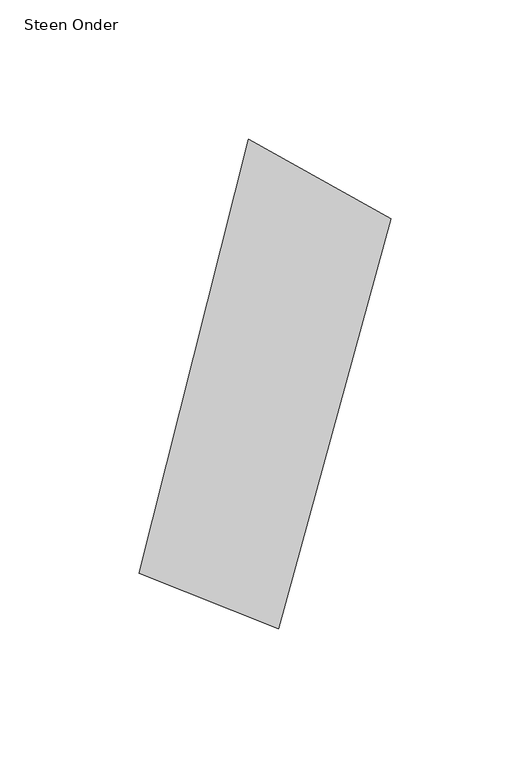
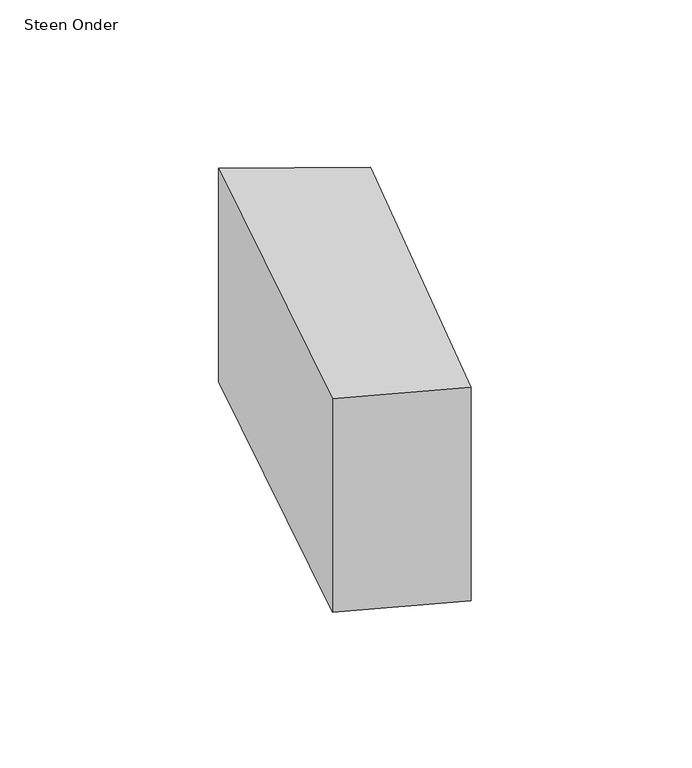
"""IFC4 building model written with IfcOpenShell, lengths in millimetres: proxy geometry, 00_GMA_steen_versie_4 : Steen Onder."""

from ifc_helpers import new_model, si_unit, origin, origin_with_axes, place, context, project, spatial, polyline, outline, extrude, source, transform, mapped, element, save


def steen_onder_9c941e0e(model_context):
    return source(origin(), model_context, "Body", "SweptSolid", [
        extrude(outline(polyline([(120.6056337, 141.9590493), (80.2980463, -4.9882444), (30.3654348, 14.8668182), (69.5288803, 170.4317439), (120.6056337, 141.9590493)])), origin_with_axes(), (0.0, 0.0, 1.0), 100.0),
    ])


if __name__ == "__main__":
    model = new_model("IFC4")
    model_context = context("Model", 3, world=origin())
    ifc_project = project(units=[si_unit("LENGTHUNIT", "METRE", prefix="MILLI")], contexts=[model_context])
    site = spatial("IfcSite", under=ifc_project)
    building = spatial("IfcBuilding", under=site)
    placement = place(None, origin())
    steen_onder_shape = steen_onder_9c941e0e(model_context)
    element("IfcBuildingElementProxy", 1, Name="00_GMA_steen_versie_4 : Steen Onder", ObjectType="00_GMA_steen_versie_4 : Steen Onder", at=placement, inside=building, context=model_context, shape_type="MappedRepresentation", body=[
        mapped(steen_onder_shape, transform((0.0, 0.0, 0.0), x_axis=(1.0, 0.0, 0.0), y_axis=(0.0, 1.0, 0.0), z_axis=(0.0, 0.0, 1.0))),
    ])
    save(model, "model.ifc")

# Revit data of these elements
# Type "00_GMA_steen_versie_4 : Steen Onder"
#   StootVoegHalfBoven [instance default] = 5 mm
#   StootVoegHalf [instance default] = 5 mm
#   StootVoegBreedteOnder = 10 mm
#   StootVoegBreedteBoven = 10 mm
#   Steendikte = 100 mm
#   LintVoegOnderHalf = 0 mm
#   LintVoegOnder = 0 mm
#   LintVoegBovenHalf = 5 mm
#   LintVoegBoven = 10 mm
#   materiaal = none
#   MateriaalVoeg = none
#   Default Elevation = 0
